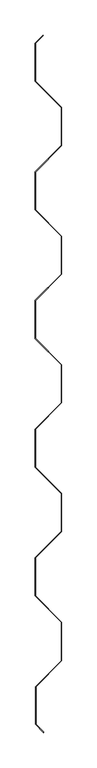
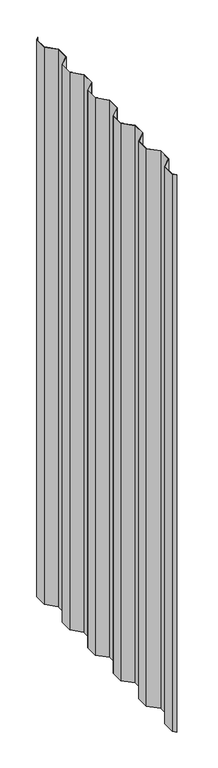
"""IFC4 building model written with IfcOpenShell, lengths in millimetres: proxy geometry, MBCI 7.2-V Panel16 : MBCI 7.2-V Panel-1."""

from ifc_helpers import new_model, si_unit, frame, origin, place, context, project, spatial, polyline, outline, extrude, source, transform, mapped, element, save


def generic_models_33612dee(model_context):
    return source(origin(), model_context, "Body", "SweptSolid", [
        extrude(outline(polyline([(590353.5827614, -533439.9919067), (590353.5827614, -533385.8801976), (590364.9833956, -533374.4795634), (590365.0253204, -533375.2795376), (590354.1780739, -533386.1267841), (590354.1780739, -533439.7453202), (590391.6684739, -533477.2357202), (590391.6684739, -533531.5163841), (590354.1780739, -533569.0067841), (590354.1780739, -533622.6253202), (590391.6684739, -533660.1157202), (590391.6684739, -533714.3963841), (590354.1780739, -533751.8867841), (590354.1780739, -533805.5053202), (590391.6684739, -533842.9957202), (590391.6684739, -533897.2763841), (590354.1780739, -533934.7667841), (590354.1780739, -533988.3853202), (590391.6684739, -534025.8757202), (590391.6684739, -534080.1563841), (590354.1780739, -534117.6467841), (590354.1780739, -534171.2653202), (590391.6684739, -534208.7557202), (590391.6684739, -534263.8999841), (590354.7876739, -534300.7807841), (590354.7876739, -534353.8689111), (590365.9181078, -534364.999345), (590365.8630841, -534365.7862203), (590354.1923614, -534354.1154976), (590354.1923614, -534300.5341976), (590391.0731614, -534263.6533976), (590391.0731614, -534209.0023067), (590353.5827614, -534171.5119067), (590353.5827614, -534117.4001976), (590391.0731614, -534079.9097976), (590391.0731614, -534026.1223067), (590353.5827614, -533988.6319067), (590353.5827614, -533934.5201976), (590391.0731614, -533897.0297976), (590391.0731614, -533843.2423067), (590353.5827614, -533805.7519067), (590353.5827614, -533751.6401976), (590391.0731614, -533714.1497976), (590391.0731614, -533660.3623067), (590353.5827614, -533622.8719067), (590353.5827614, -533568.7601976), (590391.0731614, -533531.2697976), (590391.0731614, -533477.4823067), (590353.5827614, -533439.9919067)])), frame((0.0, 0.0, 6.35), z_axis=(0.0, 0.0, 1.0), x_axis=(1.0, 0.0, 0.0)), (0.0, 0.0, 1.0), 2432.05),
    ])


if __name__ == "__main__":
    model = new_model("IFC4")
    model_context = context("Model", 3, world=origin())
    ifc_project = project(units=[si_unit("LENGTHUNIT", "METRE", prefix="MILLI")], contexts=[model_context])
    site = spatial("IfcSite", under=ifc_project)
    building = spatial("IfcBuilding", under=site)
    placement = place(None, origin())
    generic_models_shape = generic_models_33612dee(model_context)
    element("IfcBuildingElementProxy", 1, Name="MBCI 7.2-V Panel16 : MBCI 7.2-V Panel-1", ObjectType="MBCI 7.2-V Panel16 : MBCI 7.2-V Panel-1", at=placement, inside=building, context=model_context, shape_type="MappedRepresentation", body=[
        mapped(generic_models_shape, transform((0.0, 0.0, 0.0), x_axis=(1.0, 0.0, 0.0), y_axis=(0.0, 1.0, 0.0), z_axis=(0.0, 0.0, 1.0))),
    ])
    save(model, "model.ifc")

# Revit data of these elements
# Element 1 (IfcBuildingElementProxy, "MBCI 7.2-V Panel16 : MBCI 7.2-V Panel-1")
#   Materials on its faces: "MTL PANEL"
# Materials
#   "MTL PANEL": class "Generic", colour RGB 239 242 240, transparency 0, Cost = 0
